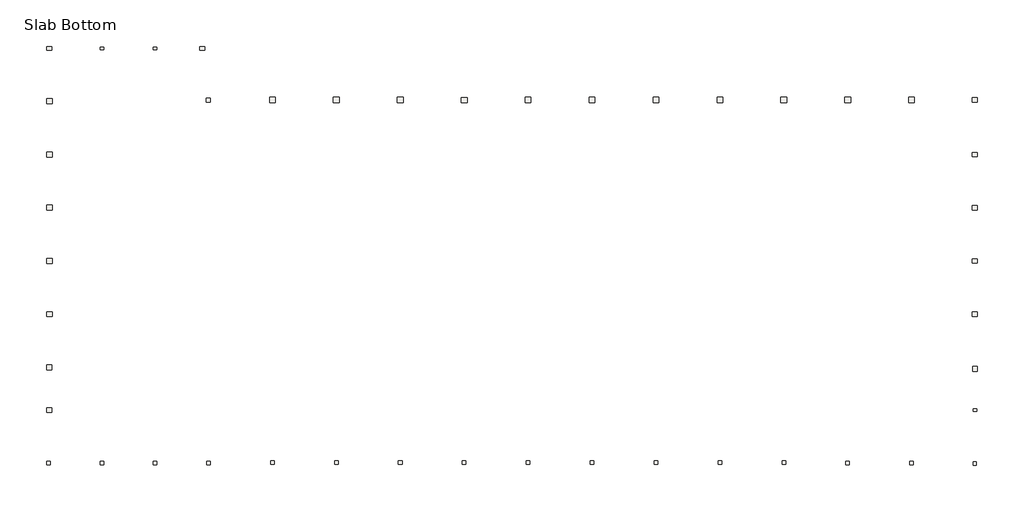
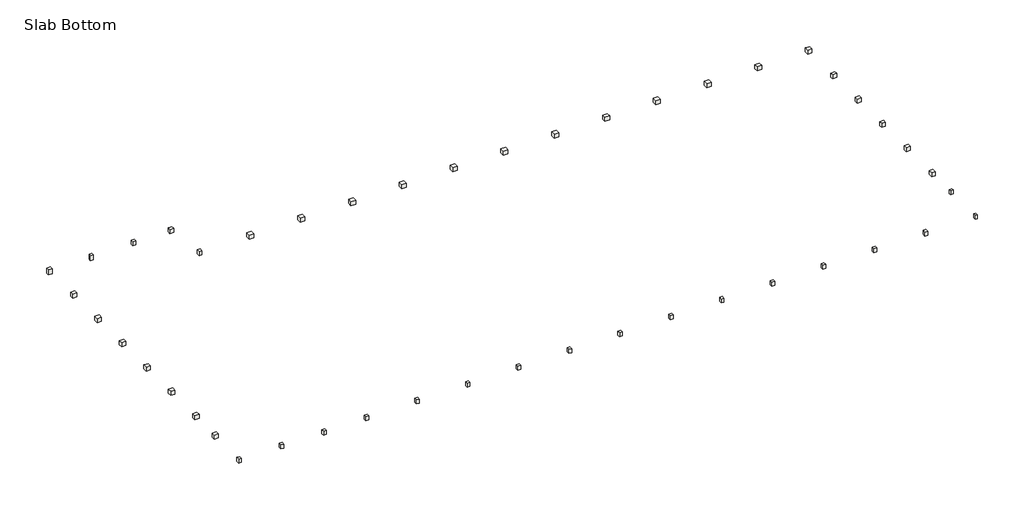
# One storey: 46 slabs.
"""IFC4 building model written with IfcOpenShell, lengths in millimetres."""

from ifc_helpers import new_model, si_unit, frame, origin, place, context, project, spatial, polyline, outline, extrude, element, save

model = new_model("IFC4")

# Units and contexts
model_context = context("Model", 3, world=origin())
ifc_project = project(units=[si_unit("LENGTHUNIT", "METRE", prefix="MILLI")], contexts=[model_context])

# Site, building, storey
site = spatial("IfcSite", under=ifc_project)
building = spatial("IfcBuilding", under=site)
storey = spatial("IfcBuildingStorey", under=building, Name="Slab Bottom", Elevation=-152.4)

# Slabs
placement = place(None, origin())
element("IfcSlab", 1, ObjectType="Footing-Rectangular : P1", at=placement, inside=storey, context=model_context, shape_type="SweptSolid", body=[
    extrude(outline(polyline([(411246.7398264, -572441.1413841), (411602.3398264, -572441.1413841), (411602.3398264, -572745.9413841), (411246.7398264, -572745.9413841), (411246.7398264, -572441.1413841)])), frame((0.0, 0.0, -914.4), z_axis=(0.0, 0.0, 1.0), x_axis=(1.0, 0.0, 0.0)), (0.0, 0.0, 1.0), 609.6),
])
element("IfcSlab", 2, ObjectType="Footing-Rectangular : P11", at=placement, inside=storey, context=model_context, shape_type="SweptSolid", body=[
    extrude(outline(polyline([(411126.0898264, -549562.0913841), (411126.0898264, -549054.0913841), (411684.8898264, -549054.0913841), (411684.8898264, -549562.0913841), (411126.0898264, -549562.0913841)])), frame((0.0, 0.0, -914.4), z_axis=(0.0, 0.0, 1.0), x_axis=(1.0, 0.0, 0.0)), (0.0, 0.0, 1.0), 609.6),
])
element("IfcSlab", 3, ObjectType="Footing-Rectangular : P11A", at=placement, inside=storey, context=model_context, shape_type="SweptSolid", body=[
    extrude(outline(polyline([(411126.0898264, -561817.5913841), (411126.0898264, -561309.5913841), (411684.8898264, -561309.5913841), (411684.8898264, -561817.5913841), (411126.0898264, -561817.5913841)])), frame((0.0, 0.0, -914.4), z_axis=(0.0, 0.0, 1.0), x_axis=(1.0, 0.0, 0.0)), (0.0, 0.0, 1.0), 609.6),
])
element("IfcSlab", 4, ObjectType="Footing-Rectangular : P12", at=placement, inside=storey, context=model_context, shape_type="SweptSolid", body=[
    extrude(outline(polyline([(304649.2898264, -537331.9913841), (304649.2898264, -536773.1913841), (305258.8898264, -536773.1913841), (305258.8898264, -537331.9913841), (304649.2898264, -537331.9913841)])), frame((0.0, 0.0, -914.4), z_axis=(0.0, 0.0, 1.0), x_axis=(1.0, 0.0, 0.0)), (0.0, 0.0, 1.0), 609.6),
])
element("IfcSlab", 5, ObjectType="Footing-Rectangular : P12", at=placement, inside=storey, context=model_context, shape_type="SweptSolid", body=[
    extrude(outline(polyline([(304649.2898264, -543459.7413841), (304649.2898264, -542900.9413841), (305258.8898264, -542900.9413841), (305258.8898264, -543459.7413841), (304649.2898264, -543459.7413841)])), frame((0.0, 0.0, -914.4), z_axis=(0.0, 0.0, 1.0), x_axis=(1.0, 0.0, 0.0)), (0.0, 0.0, 1.0), 609.6),
])
element("IfcSlab", 6, ObjectType="Footing-Rectangular : P12", at=placement, inside=storey, context=model_context, shape_type="SweptSolid", body=[
    extrude(outline(polyline([(304649.2898264, -549587.4913841), (304649.2898264, -549028.6913841), (305258.8898264, -549028.6913841), (305258.8898264, -549587.4913841), (304649.2898264, -549587.4913841)])), frame((0.0, 0.0, -914.4), z_axis=(0.0, 0.0, 1.0), x_axis=(1.0, 0.0, 0.0)), (0.0, 0.0, 1.0), 609.6),
])
element("IfcSlab", 7, ObjectType="Footing-Rectangular : P12", at=placement, inside=storey, context=model_context, shape_type="SweptSolid", body=[
    extrude(outline(polyline([(304649.2898264, -555715.2413841), (304649.2898264, -555156.4413841), (305258.8898264, -555156.4413841), (305258.8898264, -555715.2413841), (304649.2898264, -555715.2413841)])), frame((0.0, 0.0, -914.4), z_axis=(0.0, 0.0, 1.0), x_axis=(1.0, 0.0, 0.0)), (0.0, 0.0, 1.0), 609.6),
])
element("IfcSlab", 8, ObjectType="Footing-Rectangular : P12", at=placement, inside=storey, context=model_context, shape_type="SweptSolid", body=[
    extrude(outline(polyline([(304649.2898264, -561842.9913841), (304649.2898264, -561284.1913841), (305258.8898264, -561284.1913841), (305258.8898264, -561842.9913841), (304649.2898264, -561842.9913841)])), frame((0.0, 0.0, -914.4), z_axis=(0.0, 0.0, 1.0), x_axis=(1.0, 0.0, 0.0)), (0.0, 0.0, 1.0), 609.6),
])
element("IfcSlab", 9, ObjectType="Footing-Rectangular : P12", at=placement, inside=storey, context=model_context, shape_type="SweptSolid", body=[
    extrude(outline(polyline([(304623.8898264, -567970.7413841), (304623.8898264, -567411.9413841), (305233.4898264, -567411.9413841), (305233.4898264, -567970.7413841), (304623.8898264, -567970.7413841)])), frame((0.0, 0.0, -914.4), z_axis=(0.0, 0.0, 1.0), x_axis=(1.0, 0.0, 0.0)), (0.0, 0.0, 1.0), 609.6),
])
element("IfcSlab", 10, ObjectType="Footing-Rectangular : P13", at=placement, inside=storey, context=model_context, shape_type="SweptSolid", body=[
    extrude(outline(polyline([(403777.974756, -536594.2315281), (404438.374756, -536594.2315281), (404438.374756, -537203.8315281), (403777.974756, -537203.8315281), (403777.974756, -536594.2315281)])), frame((0.0, 0.0, -914.4), z_axis=(0.0, 0.0, 1.0), x_axis=(1.0, 0.0, 0.0)), (0.0, 0.0, 1.0), 609.6),
])
element("IfcSlab", 11, ObjectType="Footing-Rectangular : P13", at=placement, inside=storey, context=model_context, shape_type="SweptSolid", body=[
    extrude(outline(polyline([(396451.2398264, -536601.7413358), (397111.6398264, -536601.7413358), (397111.6398264, -537211.3413358), (396451.2398264, -537211.3413358), (396451.2398264, -536601.7413358)])), frame((0.0, 0.0, -914.4), z_axis=(0.0, 0.0, 1.0), x_axis=(1.0, 0.0, 0.0)), (0.0, 0.0, 1.0), 609.6),
])
element("IfcSlab", 12, ObjectType="Footing-Rectangular : P13", at=placement, inside=storey, context=model_context, shape_type="SweptSolid", body=[
    extrude(outline(polyline([(389097.9398264, -536601.7413358), (389758.3398264, -536601.7413358), (389758.3398264, -537211.3413358), (389097.9398264, -537211.3413358), (389097.9398264, -536601.7413358)])), frame((0.0, 0.0, -914.4), z_axis=(0.0, 0.0, 1.0), x_axis=(1.0, 0.0, 0.0)), (0.0, 0.0, 1.0), 609.6),
])
element("IfcSlab", 13, ObjectType="Footing-Rectangular : P13", at=placement, inside=storey, context=model_context, shape_type="SweptSolid", body=[
    extrude(outline(polyline([(381744.6398264, -536601.7413358), (382405.0398264, -536601.7413358), (382405.0398264, -537211.3413358), (381744.6398264, -537211.3413358), (381744.6398264, -536601.7413358)])), frame((0.0, 0.0, -914.4), z_axis=(0.0, 0.0, 1.0), x_axis=(1.0, 0.0, 0.0)), (0.0, 0.0, 1.0), 609.6),
])
element("IfcSlab", 14, ObjectType="Footing-Rectangular : P13", at=placement, inside=storey, context=model_context, shape_type="SweptSolid", body=[
    extrude(outline(polyline([(374391.3398264, -536601.7413358), (375051.7398264, -536601.7413358), (375051.7398264, -537211.3413358), (374391.3398264, -537211.3413358), (374391.3398264, -536601.7413358)])), frame((0.0, 0.0, -914.4), z_axis=(0.0, 0.0, 1.0), x_axis=(1.0, 0.0, 0.0)), (0.0, 0.0, 1.0), 609.6),
])
element("IfcSlab", 15, ObjectType="Footing-Rectangular : P13", at=placement, inside=storey, context=model_context, shape_type="SweptSolid", body=[
    extrude(outline(polyline([(367038.0398264, -536601.7413358), (367698.4398264, -536601.7413358), (367698.4398264, -537211.3413358), (367038.0398264, -537211.3413358), (367038.0398264, -536601.7413358)])), frame((0.0, 0.0, -914.4), z_axis=(0.0, 0.0, 1.0), x_axis=(1.0, 0.0, 0.0)), (0.0, 0.0, 1.0), 609.6),
])
element("IfcSlab", 16, ObjectType="Footing-Rectangular : P13", at=placement, inside=storey, context=model_context, shape_type="SweptSolid", body=[
    extrude(outline(polyline([(359684.7398264, -536601.7413358), (360345.1398264, -536601.7413358), (360345.1398264, -537211.3413358), (359684.7398264, -537211.3413358), (359684.7398264, -536601.7413358)])), frame((0.0, 0.0, -914.4), z_axis=(0.0, 0.0, 1.0), x_axis=(1.0, 0.0, 0.0)), (0.0, 0.0, 1.0), 609.6),
])
element("IfcSlab", 17, ObjectType="Footing-Rectangular : P13", at=placement, inside=storey, context=model_context, shape_type="SweptSolid", body=[
    extrude(outline(polyline([(352331.4398264, -536614.4413358), (352991.8398264, -536614.4413358), (352991.8398264, -537224.0413358), (352331.4398264, -537224.0413358), (352331.4398264, -536614.4413358)])), frame((0.0, 0.0, -914.4), z_axis=(0.0, 0.0, 1.0), x_axis=(1.0, 0.0, 0.0)), (0.0, 0.0, 1.0), 609.6),
])
element("IfcSlab", 18, ObjectType="Footing-Rectangular : P13", at=placement, inside=storey, context=model_context, shape_type="SweptSolid", body=[
    extrude(outline(polyline([(344978.1398264, -536601.7413358), (345638.5398264, -536601.7413358), (345638.5398264, -537211.3413358), (344978.1398264, -537211.3413358), (344978.1398264, -536601.7413358)])), frame((0.0, 0.0, -914.4), z_axis=(0.0, 0.0, 1.0), x_axis=(1.0, 0.0, 0.0)), (0.0, 0.0, 1.0), 609.6),
])
element("IfcSlab", 19, ObjectType="Footing-Rectangular : P13", at=placement, inside=storey, context=model_context, shape_type="SweptSolid", body=[
    extrude(outline(polyline([(337624.8398264, -536601.7413358), (338285.2398264, -536601.7413358), (338285.2398264, -537211.3413358), (337624.8398264, -537211.3413358), (337624.8398264, -536601.7413358)])), frame((0.0, 0.0, -914.4), z_axis=(0.0, 0.0, 1.0), x_axis=(1.0, 0.0, 0.0)), (0.0, 0.0, 1.0), 609.6),
])
element("IfcSlab", 20, ObjectType="Footing-Rectangular : P13", at=placement, inside=storey, context=model_context, shape_type="SweptSolid", body=[
    extrude(outline(polyline([(330271.5398264, -536601.7413358), (330931.9398264, -536601.7413358), (330931.9398264, -537211.3413358), (330271.5398264, -537211.3413358), (330271.5398264, -536601.7413358)])), frame((0.0, 0.0, -914.4), z_axis=(0.0, 0.0, 1.0), x_axis=(1.0, 0.0, 0.0)), (0.0, 0.0, 1.0), 609.6),
])
element("IfcSlab", 21, ObjectType="Footing-Rectangular : P13A", at=placement, inside=storey, context=model_context, shape_type="SweptSolid", body=[
    extrude(outline(polyline([(411094.3398264, -536620.7913358), (411703.9398264, -536620.7913358), (411703.9398264, -537179.5913358), (411094.3398264, -537179.5913358), (411094.3398264, -536620.7913358)])), frame((0.0, 0.0, -914.4), z_axis=(0.0, 0.0, 1.0), x_axis=(1.0, 0.0, 0.0)), (0.0, 0.0, 1.0), 609.6),
])
element("IfcSlab", 22, ObjectType="Footing-Rectangular : P14", at=placement, inside=storey, context=model_context, shape_type="SweptSolid", body=[
    extrude(outline(polyline([(304649.2898264, -572847.5413841), (304649.2898264, -572339.5413841), (305208.0898264, -572339.5413841), (305208.0898264, -572847.5413841), (304649.2898264, -572847.5413841)])), frame((0.0, 0.0, -914.4), z_axis=(0.0, 0.0, 1.0), x_axis=(1.0, 0.0, 0.0)), (0.0, 0.0, 1.0), 609.6),
])
element("IfcSlab", 23, ObjectType="Footing-Rectangular : P2", at=placement, inside=storey, context=model_context, shape_type="SweptSolid", body=[
    extrude(outline(polyline([(322797.5898264, -530747.0413841), (322797.5898264, -531153.4413841), (322238.7898264, -531153.4413841), (322238.7898264, -530747.0413841), (322797.5898264, -530747.0413841)])), frame((0.0, 0.0, -914.4), z_axis=(0.0, 0.0, 1.0), x_axis=(1.0, 0.0, 0.0)), (0.0, 0.0, 1.0), 609.6),
])
element("IfcSlab", 24, ObjectType="Footing-Rectangular : P3", at=placement, inside=storey, context=model_context, shape_type="SweptSolid", body=[
    extrude(outline(polyline([(411246.7398264, -578543.4913841), (411551.5398264, -578543.4913841), (411551.5398264, -578949.8913841), (411246.7398264, -578949.8913841), (411246.7398264, -578543.4913841)])), frame((0.0, 0.0, -914.4), z_axis=(0.0, 0.0, 1.0), x_axis=(1.0, 0.0, 0.0)), (0.0, 0.0, 1.0), 609.6),
])
element("IfcSlab", 25, ObjectType="Footing-Rectangular : P4", at=placement, inside=storey, context=model_context, shape_type="SweptSolid", body=[
    extrude(outline(polyline([(310789.7398264, -531108.9913841), (310789.7398264, -530804.1913841), (311196.1398264, -530804.1913841), (311196.1398264, -531108.9913841), (310789.7398264, -531108.9913841)])), frame((0.0, 0.0, -1066.8), z_axis=(0.0, 0.0, 1.0), x_axis=(1.0, 0.0, 0.0)), (0.0, 0.0, 1.0), 762.0),
])
element("IfcSlab", 26, ObjectType="Footing-Rectangular : P4", at=placement, inside=storey, context=model_context, shape_type="SweptSolid", body=[
    extrude(outline(polyline([(317323.8898264, -531108.9913841), (316917.4898264, -531108.9913841), (316917.4898264, -530804.1913841), (317323.8898264, -530804.1913841), (317323.8898264, -531108.9913841)])), frame((0.0, 0.0, -914.4), z_axis=(0.0, 0.0, 1.0), x_axis=(1.0, 0.0, 0.0)), (0.0, 0.0, 1.0), 609.6),
])
element("IfcSlab", 27, ObjectType="Footing-Rectangular : P5", at=placement, inside=storey, context=model_context, shape_type="SweptSolid", body=[
    extrude(outline(polyline([(311196.1398264, -578892.7413841), (310789.7398264, -578892.7413841), (310789.7398264, -578486.3413841), (311196.1398264, -578486.3413841), (311196.1398264, -578892.7413841)])), frame((0.0, 0.0, -914.4), z_axis=(0.0, 0.0, 1.0), x_axis=(1.0, 0.0, 0.0)), (0.0, 0.0, 1.0), 609.6),
])
element("IfcSlab", 28, ObjectType="Footing-Rectangular : P5", at=placement, inside=storey, context=model_context, shape_type="SweptSolid", body=[
    extrude(outline(polyline([(317327.0648264, -578937.1913841), (316920.6648264, -578937.1913841), (316920.6648264, -578530.7913841), (317327.0648264, -578530.7913841), (317327.0648264, -578937.1913841)])), frame((0.0, 0.0, -914.4), z_axis=(0.0, 0.0, 1.0), x_axis=(1.0, 0.0, 0.0)), (0.0, 0.0, 1.0), 609.6),
])
element("IfcSlab", 29, ObjectType="Footing-Rectangular : P5", at=placement, inside=storey, context=model_context, shape_type="SweptSolid", body=[
    extrude(outline(polyline([(330398.5398264, -578448.2413841), (330804.9398264, -578448.2413841), (330804.9398264, -578854.6413841), (330398.5398264, -578854.6413841), (330398.5398264, -578448.2413841)])), frame((0.0, 0.0, -914.4), z_axis=(0.0, 0.0, 1.0), x_axis=(1.0, 0.0, 0.0)), (0.0, 0.0, 1.0), 609.6),
])
element("IfcSlab", 30, ObjectType="Footing-Rectangular : P5", at=placement, inside=storey, context=model_context, shape_type="SweptSolid", body=[
    extrude(outline(polyline([(337751.8398264, -578448.2413841), (338158.2398264, -578448.2413841), (338158.2398264, -578854.6413841), (337751.8398264, -578854.6413841), (337751.8398264, -578448.2413841)])), frame((0.0, 0.0, -914.4), z_axis=(0.0, 0.0, 1.0), x_axis=(1.0, 0.0, 0.0)), (0.0, 0.0, 1.0), 609.6),
])
element("IfcSlab", 31, ObjectType="Footing-Rectangular : P5", at=placement, inside=storey, context=model_context, shape_type="SweptSolid", body=[
    extrude(outline(polyline([(345105.1398264, -578448.2413841), (345511.5398264, -578448.2413841), (345511.5398264, -578854.6413841), (345105.1398264, -578854.6413841), (345105.1398264, -578448.2413841)])), frame((0.0, 0.0, -914.4), z_axis=(0.0, 0.0, 1.0), x_axis=(1.0, 0.0, 0.0)), (0.0, 0.0, 1.0), 609.6),
])
element("IfcSlab", 32, ObjectType="Footing-Rectangular : P5", at=placement, inside=storey, context=model_context, shape_type="SweptSolid", body=[
    extrude(outline(polyline([(352458.4398264, -578448.2413841), (352864.8398264, -578448.2413841), (352864.8398264, -578854.6413841), (352458.4398264, -578854.6413841), (352458.4398264, -578448.2413841)])), frame((0.0, 0.0, -914.4), z_axis=(0.0, 0.0, 1.0), x_axis=(1.0, 0.0, 0.0)), (0.0, 0.0, 1.0), 609.6),
])
element("IfcSlab", 33, ObjectType="Footing-Rectangular : P5", at=placement, inside=storey, context=model_context, shape_type="SweptSolid", body=[
    extrude(outline(polyline([(359811.7398264, -578448.2413841), (360218.1398264, -578448.2413841), (360218.1398264, -578854.6413841), (359811.7398264, -578854.6413841), (359811.7398264, -578448.2413841)])), frame((0.0, 0.0, -914.4), z_axis=(0.0, 0.0, 1.0), x_axis=(1.0, 0.0, 0.0)), (0.0, 0.0, 1.0), 609.6),
])
element("IfcSlab", 34, ObjectType="Footing-Rectangular : P5", at=placement, inside=storey, context=model_context, shape_type="SweptSolid", body=[
    extrude(outline(polyline([(367165.0398264, -578448.2413841), (367571.4398264, -578448.2413841), (367571.4398264, -578854.6413841), (367165.0398264, -578854.6413841), (367165.0398264, -578448.2413841)])), frame((0.0, 0.0, -914.4), z_axis=(0.0, 0.0, 1.0), x_axis=(1.0, 0.0, 0.0)), (0.0, 0.0, 1.0), 609.6),
])
element("IfcSlab", 35, ObjectType="Footing-Rectangular : P5", at=placement, inside=storey, context=model_context, shape_type="SweptSolid", body=[
    extrude(outline(polyline([(374518.3398264, -578448.2413841), (374924.7398264, -578448.2413841), (374924.7398264, -578854.6413841), (374518.3398264, -578854.6413841), (374518.3398264, -578448.2413841)])), frame((0.0, 0.0, -914.4), z_axis=(0.0, 0.0, 1.0), x_axis=(1.0, 0.0, 0.0)), (0.0, 0.0, 1.0), 609.6),
])
element("IfcSlab", 36, ObjectType="Footing-Rectangular : P5", at=placement, inside=storey, context=model_context, shape_type="SweptSolid", body=[
    extrude(outline(polyline([(381871.6398264, -578448.2413841), (382278.0398264, -578448.2413841), (382278.0398264, -578854.6413841), (381871.6398264, -578854.6413841), (381871.6398264, -578448.2413841)])), frame((0.0, 0.0, -914.4), z_axis=(0.0, 0.0, 1.0), x_axis=(1.0, 0.0, 0.0)), (0.0, 0.0, 1.0), 609.6),
])
element("IfcSlab", 37, ObjectType="Footing-Rectangular : P5", at=placement, inside=storey, context=model_context, shape_type="SweptSolid", body=[
    extrude(outline(polyline([(389224.9398264, -578448.2413841), (389631.3398264, -578448.2413841), (389631.3398264, -578854.6413841), (389224.9398264, -578854.6413841), (389224.9398264, -578448.2413841)])), frame((0.0, 0.0, -914.4), z_axis=(0.0, 0.0, 1.0), x_axis=(1.0, 0.0, 0.0)), (0.0, 0.0, 1.0), 609.6),
])
element("IfcSlab", 38, ObjectType="Footing-Rectangular : P5", at=placement, inside=storey, context=model_context, shape_type="SweptSolid", body=[
    extrude(outline(polyline([(403931.5398264, -578530.7913841), (404337.9398264, -578530.7913841), (404337.9398264, -578937.1913841), (403931.5398264, -578937.1913841), (403931.5398264, -578530.7913841)])), frame((0.0, 0.0, -914.4), z_axis=(0.0, 0.0, 1.0), x_axis=(1.0, 0.0, 0.0)), (0.0, 0.0, 1.0), 609.6),
])
element("IfcSlab", 39, ObjectType="Footing-Rectangular : P5A", at=placement, inside=storey, context=model_context, shape_type="SweptSolid", body=[
    extrude(outline(polyline([(396578.2398264, -578530.7913841), (396984.6398264, -578530.7913841), (396984.6398264, -578937.1913841), (396578.2398264, -578937.1913841), (396578.2398264, -578530.7913841)])), frame((0.0, 0.0, -914.4), z_axis=(0.0, 0.0, 1.0), x_axis=(1.0, 0.0, 0.0)), (0.0, 0.0, 1.0), 609.6),
])
element("IfcSlab", 40, ObjectType="Footing-Rectangular : P5B", at=placement, inside=storey, context=model_context, shape_type="SweptSolid", body=[
    extrude(outline(polyline([(323064.2898264, -578899.0913841), (323064.2898264, -578492.6913841), (323470.6898264, -578492.6913841), (323470.6898264, -578899.0913841), (323064.2898264, -578899.0913841)])), frame((0.0, 0.0, -914.4), z_axis=(0.0, 0.0, 1.0), x_axis=(1.0, 0.0, 0.0)), (0.0, 0.0, 1.0), 609.6),
])
element("IfcSlab", 41, ObjectType="Footing-Rectangular : P5C", at=placement, inside=storey, context=model_context, shape_type="SweptSolid", body=[
    extrude(outline(polyline([(304642.9398264, -578899.0913841), (304642.9398264, -578492.6913841), (305049.3398264, -578492.6913841), (305049.3398264, -578899.0913841), (304642.9398264, -578899.0913841)])), frame((0.0, 0.0, -914.4), z_axis=(0.0, 0.0, 1.0), x_axis=(1.0, 0.0, 0.0)), (0.0, 0.0, 1.0), 609.6),
])
element("IfcSlab", 42, ObjectType="Footing-Rectangular : P6", at=placement, inside=storey, context=model_context, shape_type="SweptSolid", body=[
    extrude(outline(polyline([(323019.8398264, -536722.3913841), (323426.2398264, -536722.3913841), (323426.2398264, -537179.5913841), (323019.8398264, -537179.5913841), (323019.8398264, -536722.3913841)])), frame((0.0, 0.0, -914.4), z_axis=(0.0, 0.0, 1.0), x_axis=(1.0, 0.0, 0.0)), (0.0, 0.0, 1.0), 609.6),
])
element("IfcSlab", 43, ObjectType="Footing-Rectangular : P6A", at=placement, inside=storey, context=model_context, shape_type="SweptSolid", body=[
    extrude(outline(polyline([(304655.6398264, -530747.0413841), (305214.4398264, -530747.0413841), (305214.4398264, -531153.4413841), (304655.6398264, -531153.4413841), (304655.6398264, -530747.0413841)])), frame((0.0, 0.0, -1066.8), z_axis=(0.0, 0.0, 1.0), x_axis=(1.0, 0.0, 0.0)), (0.0, 0.0, 1.0), 762.0),
])
element("IfcSlab", 44, ObjectType="Footing-Rectangular : P7", at=placement, inside=storey, context=model_context, shape_type="SweptSolid", body=[
    extrude(outline(polyline([(411145.1398264, -567577.0413841), (411653.1398264, -567577.0413841), (411653.1398264, -568135.8413841), (411145.1398264, -568135.8413841), (411145.1398264, -567577.0413841)])), frame((0.0, 0.0, -914.4), z_axis=(0.0, 0.0, 1.0), x_axis=(1.0, 0.0, 0.0)), (0.0, 0.0, 1.0), 609.6),
])
element("IfcSlab", 45, ObjectType="Footing-Rectangular : P8", at=placement, inside=storey, context=model_context, shape_type="SweptSolid", body=[
    extrude(outline(polyline([(411126.0898264, -555664.4413841), (411126.0898264, -555207.2413841), (411684.8898264, -555207.2413841), (411684.8898264, -555664.4413841), (411126.0898264, -555664.4413841)])), frame((0.0, 0.0, -914.4), z_axis=(0.0, 0.0, 1.0), x_axis=(1.0, 0.0, 0.0)), (0.0, 0.0, 1.0), 609.6),
])
element("IfcSlab", 46, ObjectType="Footing-Rectangular : P9", at=placement, inside=storey, context=model_context, shape_type="SweptSolid", body=[
    extrude(outline(polyline([(411094.3398264, -543408.9413841), (411094.3398264, -542951.7413841), (411703.9398264, -542951.7413841), (411703.9398264, -543408.9413841), (411094.3398264, -543408.9413841)])), frame((0.0, 0.0, -914.4), z_axis=(0.0, 0.0, 1.0), x_axis=(1.0, 0.0, 0.0)), (0.0, 0.0, 1.0), 609.6),
])

save(model, "model.ifc")

# Revit data of these elements
# Type "Footing-Rectangular : P1"
#   Type Mark = ""
#   Assembly Code = "A1010100"
#   Width = 1' - 2"
#   Length = 1' - 0"
#   Thickness = 2' - 6"
#   Structural Material [instance default] = CONCRETE FOOTING - SEE STRUCT DWGS.
# Type "Footing-Rectangular : P11"
#   Assembly Code = "A1010100"
#   Width = 1' - 8"
#   Length = 1' - 10"
#   Thickness = 2' - 6"
#   Structural Material [instance default] = CONCRETE FOOTING - SEE STRUCT DWGS.
# Type "Footing-Rectangular : P11A"
#   Assembly Code = "A1010100"
#   Width = 1' - 8"
#   Length = 1' - 10"
#   Thickness = 2' - 6"
#   Structural Material [instance default] = CONCRETE FOOTING - SEE STRUCT DWGS.
# Type "Footing-Rectangular : P12"
#   Assembly Code = "A1010100"
#   Width = 1' - 10"
#   Length = 2' - 0"
#   Thickness = 2' - 6"
#   Structural Material [instance default] = CONCRETE FOOTING - SEE STRUCT DWGS.
# Type "Footing-Rectangular : P13"
#   Assembly Code = "A1010100"
#   Width = 2' - 2"
#   Length = 2' - 0"
#   Thickness = 2' - 6"
#   Structural Material [instance default] = CONCRETE FOOTING - SEE STRUCT DWGS.
# Type "Footing-Rectangular : P13A"
#   Assembly Code = "A1010100"
#   Width = 2' - 0"
#   Length = 1' - 10"
#   Thickness = 2' - 6"
#   Structural Material [instance default] = CONCRETE FOOTING - SEE STRUCT DWGS.
# Type "Footing-Rectangular : P14"
#   Assembly Code = "A1010100"
#   Width = 1' - 8"
#   Length = 1' - 10"
#   Thickness = 2' - 6"
#   Structural Material [instance default] = CONCRETE FOOTING - SEE STRUCT DWGS.
# Type "Footing-Rectangular : P2"
#   Assembly Code = "A1010100"
#   Width = 1' - 4"
#   Length = 1' - 10"
#   Thickness = 2' - 6"
#   Structural Material [instance default] = CONCRETE FOOTING - SEE STRUCT DWGS.
# Type "Footing-Rectangular : P3"
#   Assembly Code = "A1010100"
#   Width = 1' - 0"
#   Length = 1' - 4"
#   Thickness = 2' - 6"
#   Structural Material [instance default] = CONCRETE FOOTING - SEE STRUCT DWGS.
# Type "Footing-Rectangular : P4"
#   Assembly Code = "A1010100"
#   Width = 1' - 4"
#   Length = 1' - 0"
#   Thickness = 2' - 6"
#   Structural Material [instance default] = CONCRETE FOOTING - SEE STRUCT DWGS.
# Type "Footing-Rectangular : P5"
#   Assembly Code = "A1010100"
#   Width = 1' - 4"
#   Length = 1' - 4"
#   Thickness = 2' - 6"
#   Structural Material [instance default] = CONCRETE FOOTING - SEE STRUCT DWGS.
# Type "Footing-Rectangular : P5A"
#   Assembly Code = "A1010100"
#   Width = 1' - 4"
#   Length = 1' - 4"
#   Thickness = 2' - 6"
#   Structural Material [instance default] = CONCRETE FOOTING - SEE STRUCT DWGS.
# Type "Footing-Rectangular : P5B"
#   Assembly Code = "A1010100"
#   Width = 1' - 4"
#   Length = 1' - 4"
#   Thickness = 2' - 6"
#   Structural Material [instance default] = CONCRETE FOOTING - SEE STRUCT DWGS.
# Type "Footing-Rectangular : P5C"
#   Assembly Code = "A1010100"
#   Width = 1' - 4"
#   Length = 1' - 4"
#   Thickness = 2' - 6"
#   Structural Material [instance default] = CONCRETE FOOTING - SEE STRUCT DWGS.
# Type "Footing-Rectangular : P6"
#   Assembly Code = "A1010100"
#   Width = 1' - 4"
#   Length = 1' - 6"
#   Thickness = 2' - 6"
#   Structural Material [instance default] = CONCRETE FOOTING - SEE STRUCT DWGS.
# Type "Footing-Rectangular : P6A"
#   Assembly Code = "A1010100"
#   Width = 1' - 4"
#   Length = 1' - 10"
#   Thickness = 2' - 6"
#   Structural Material [instance default] = CONCRETE FOOTING - SEE STRUCT DWGS.
# Type "Footing-Rectangular : P7"
#   Assembly Code = "A1010100"
#   Width = 1' - 8"
#   Length = 1' - 10"
#   Thickness = 2' - 6"
#   Structural Material [instance default] = CONCRETE FOOTING - SEE STRUCT DWGS.
# Type "Footing-Rectangular : P8"
#   Assembly Code = "A1010100"
#   Width = 1' - 6"
#   Length = 1' - 10"
#   Thickness = 2' - 6"
#   Structural Material [instance default] = CONCRETE FOOTING - SEE STRUCT DWGS.
# Type "Footing-Rectangular : P9"
#   Assembly Code = "A1010100"
#   Width = 1' - 6"
#   Length = 2' - 0"
#   Thickness = 2' - 6"
#   Structural Material [instance default] = CONCRETE FOOTING - SEE STRUCT DWGS.
# Element 1 (IfcSlab, "Footing-Rectangular : P1")
#   Comments = ""
#   Structural Material = CONCRETE PIER- SEE STRUCT DWGS.
#   Phase Created = Existing
#   Materials on its faces: "CONCRETE PIER- SEE STRUCT DWGS.", "CONCRETE FOOTING - SEE STRUCT DWGS."
# Element 2 (IfcSlab, "Footing-Rectangular : P11")
#   Comments = ""
#   Structural Material = CONCRETE PIER- SEE STRUCT DWGS.
#   Phase Created = Existing
#   Materials on its faces: "CONCRETE PIER- SEE STRUCT DWGS.", "CONCRETE FOOTING - SEE STRUCT DWGS."
# Element 3 (IfcSlab, "Footing-Rectangular : P11A")
#   Comments = ""
#   Structural Material = CONCRETE PIER- SEE STRUCT DWGS.
#   Phase Created = Existing
#   Materials on its faces: "CONCRETE PIER- SEE STRUCT DWGS.", "CONCRETE FOOTING - SEE STRUCT DWGS."
# Elements 4, 5, 6, 7, 8, 9 (IfcSlab, "Footing-Rectangular : P12")
#   Comments = ""
#   Structural Material = CONCRETE PIER- SEE STRUCT DWGS.
#   Phase Created = Existing
#   Materials on its faces: "CONCRETE PIER- SEE STRUCT DWGS.", "CONCRETE FOOTING - SEE STRUCT DWGS."
# Elements 10, 11, 12, 13, 14, 15, 16, 17, 18, 19, 20 (IfcSlab, "Footing-Rectangular : P13")
#   Comments = ""
#   Structural Material = CONCRETE PIER- SEE STRUCT DWGS.
#   Phase Created = Existing
#   Materials on its faces: "CONCRETE PIER- SEE STRUCT DWGS.", "CONCRETE FOOTING - SEE STRUCT DWGS."
# Element 21 (IfcSlab, "Footing-Rectangular : P13A")
#   Comments = ""
#   Structural Material = CONCRETE PIER- SEE STRUCT DWGS.
#   Phase Created = Existing
#   Materials on its faces: "CONCRETE PIER- SEE STRUCT DWGS.", "CONCRETE FOOTING - SEE STRUCT DWGS."
# Element 22 (IfcSlab, "Footing-Rectangular : P14")
#   Comments = ""
#   Structural Material = CONCRETE PIER- SEE STRUCT DWGS.
#   Phase Created = Existing
#   Materials on its faces: "CONCRETE PIER- SEE STRUCT DWGS.", "CONCRETE FOOTING - SEE STRUCT DWGS."
# Element 23 (IfcSlab, "Footing-Rectangular : P2")
#   Comments = ""
#   Structural Material = CONCRETE PIER- SEE STRUCT DWGS.
#   Phase Created = Existing
#   Materials on its faces: "CONCRETE PIER- SEE STRUCT DWGS.", "CONCRETE FOOTING - SEE STRUCT DWGS."
# Element 24 (IfcSlab, "Footing-Rectangular : P3")
#   Comments = ""
#   Structural Material = CONCRETE PIER- SEE STRUCT DWGS.
#   Phase Created = Existing
#   Materials on its faces: "CONCRETE PIER- SEE STRUCT DWGS.", "CONCRETE FOOTING - SEE STRUCT DWGS."
# Element 25 (IfcSlab, "Footing-Rectangular : P4")
#   Comments = ""
#   Structural Material = CONCRETE PIER- SEE STRUCT DWGS.
#   Phase Created = Existing
#   Materials on its faces: "CONCRETE PIER- SEE STRUCT DWGS."
# Element 26 (IfcSlab, "Footing-Rectangular : P4")
#   Comments = ""
#   Structural Material = CONCRETE PIER- SEE STRUCT DWGS.
#   Phase Created = Existing
#   Materials on its faces: "CONCRETE PIER- SEE STRUCT DWGS.", "CONCRETE FOOTING - SEE STRUCT DWGS."
# Elements 27, 28, 29, 30, 31, 32, 33, 34, 35, 36, 37, 38 (IfcSlab, "Footing-Rectangular : P5")
#   Comments = ""
#   Structural Material = CONCRETE PIER- SEE STRUCT DWGS.
#   Phase Created = Existing
#   Materials on its faces: "CONCRETE PIER- SEE STRUCT DWGS.", "CONCRETE FOOTING - SEE STRUCT DWGS."
# Element 39 (IfcSlab, "Footing-Rectangular : P5A")
#   Comments = ""
#   Structural Material = CONCRETE PIER- SEE STRUCT DWGS.
#   Phase Created = Existing
#   Materials on its faces: "CONCRETE PIER- SEE STRUCT DWGS.", "CONCRETE FOOTING - SEE STRUCT DWGS."
# Element 40 (IfcSlab, "Footing-Rectangular : P5B")
#   Comments = ""
#   Structural Material = CONCRETE PIER- SEE STRUCT DWGS.
#   Phase Created = Existing
#   Materials on its faces: "CONCRETE PIER- SEE STRUCT DWGS.", "CONCRETE FOOTING - SEE STRUCT DWGS."
# Element 41 (IfcSlab, "Footing-Rectangular : P5C")
#   Comments = ""
#   Structural Material = CONCRETE PIER- SEE STRUCT DWGS.
#   Phase Created = Existing
#   Materials on its faces: "CONCRETE PIER- SEE STRUCT DWGS.", "CONCRETE FOOTING - SEE STRUCT DWGS."
# Element 42 (IfcSlab, "Footing-Rectangular : P6")
#   Comments = ""
#   Structural Material = CONCRETE PIER- SEE STRUCT DWGS.
#   Phase Created = Existing
#   Materials on its faces: "CONCRETE PIER- SEE STRUCT DWGS.", "CONCRETE FOOTING - SEE STRUCT DWGS."
# Element 43 (IfcSlab, "Footing-Rectangular : P6A")
#   Comments = ""
#   Structural Material = CONCRETE PIER- SEE STRUCT DWGS.
#   Phase Created = Existing
#   Materials on its faces: "CONCRETE PIER- SEE STRUCT DWGS."
# Element 44 (IfcSlab, "Footing-Rectangular : P7")
#   Comments = ""
#   Structural Material = CONCRETE PIER- SEE STRUCT DWGS.
#   Phase Created = Existing
#   Materials on its faces: "CONCRETE PIER- SEE STRUCT DWGS.", "CONCRETE FOOTING - SEE STRUCT DWGS."
# Element 45 (IfcSlab, "Footing-Rectangular : P8")
#   Comments = ""
#   Structural Material = CONCRETE PIER- SEE STRUCT DWGS.
#   Phase Created = Existing
#   Materials on its faces: "CONCRETE PIER- SEE STRUCT DWGS.", "CONCRETE FOOTING - SEE STRUCT DWGS."
# Element 46 (IfcSlab, "Footing-Rectangular : P9")
#   Comments = ""
#   Structural Material = CONCRETE PIER- SEE STRUCT DWGS.
#   Phase Created = Existing
#   Materials on its faces: "CONCRETE PIER- SEE STRUCT DWGS.", "CONCRETE FOOTING - SEE STRUCT DWGS."
# Materials
#   "CONCRETE FOOTING - SEE STRUCT DWGS.": class "Concrete", colour RGB 192 192 192, transparency 0, Description = "Cast-in-place concrete", Cost = 0
#   "CONCRETE PIER- SEE STRUCT DWGS.": class "Concrete", colour RGB 192 192 192, transparency 0, Description = "Cast-in-place concrete", Cost = 0
